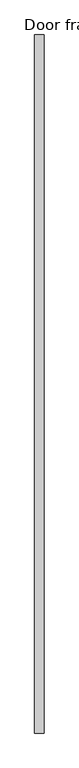
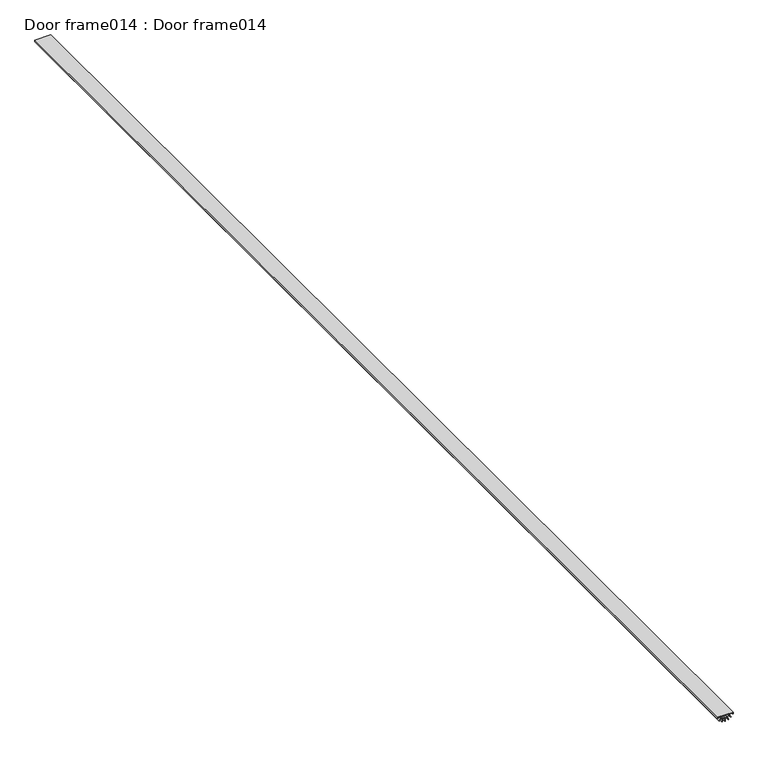
"""IFC4 building model written with IfcOpenShell, lengths in millimetres: proxy geometry, Door frame014 : Door frame014."""

import ifcopenshell
import ifcopenshell.guid

model = None  # the IFC model being written
_history = None  # IfcOwnerHistory: only IFC2X3 demands one
_inside = {}  # id of a spatial element -> (the spatial element, [elements in it])
_under = {}  # id of a project, library or spatial element -> (it, [spatial elements below it])
_declared = {}  # id of a project -> (the project, [libraries it declares])
_typed = {}  # id of a type object -> (the type object, [elements of that type])
_made_of = {}  # id of a material, layer set ... -> (it, [elements and type objects made of it])


def new_model(schema):
    """Start an empty IFC model of exactly this schema.

    Asked for "IFC4X3", IfcOpenShell would pick the latest addendum, in which some entities
    have other attributes; the version numbers below select the first issue.
    IFC2X3 requires an IfcOwnerHistory on every rooted entity: one is made here for all.
    """
    global model, _history
    if schema == "IFC4X3":
        model = ifcopenshell.file(schema_version=(4, 3, 0, 0))
    else:
        model = ifcopenshell.file(schema=schema)
    _inside.clear()
    _under.clear()
    _declared.clear()
    _typed.clear()
    _made_of.clear()
    _history = None
    if model.schema == "IFC2X3":
        org = make("IfcOrganization", Name="unknown")
        user = make(
            "IfcPersonAndOrganization",
            ThePerson=make("IfcPerson", FamilyName="unknown"),
            TheOrganization=org,
        )
        app = make(
            "IfcApplication",
            ApplicationDeveloper=org,
            Version="unknown",
            ApplicationFullName="unknown",
            ApplicationIdentifier="unknown",
        )
        _history = make(
            "IfcOwnerHistory",
            OwningUser=user,
            OwningApplication=app,
            ChangeAction="ADDED",
            CreationDate=0,
        )
    return model


def make(cls, **values):
    """One entity of the class cls with the attributes given. An attribute that is None is left unset."""
    return model.create_entity(
        cls, **{name: value for name, value in values.items() if value is not None}
    )


def rooted(cls, **values):
    """An entity with a GlobalId (a new one), such as an element, a storey or a relation."""
    return make(cls, GlobalId=ifcopenshell.guid.new(), OwnerHistory=_history, **values)


def si_unit(unit_type, name, prefix=None):
    """IfcSIUnit, for example si_unit("LENGTHUNIT", "METRE", prefix="MILLI")."""
    return make("IfcSIUnit", UnitType=unit_type, Prefix=prefix, Name=name)


def assignment(units):
    """IfcUnitAssignment: the units of a project."""
    return None if units is None else make("IfcUnitAssignment", Units=units)


def point(xyz):
    """IfcCartesianPoint."""
    return None if xyz is None else make("IfcCartesianPoint", Coordinates=xyz)


def direction(xyz):
    """IfcDirection."""
    return None if xyz is None else make("IfcDirection", DirectionRatios=xyz)


def frame(location, z_axis=None, x_axis=None):
    """IfcAxis2Placement3D, a coordinate frame: its origin and axes. An axis left out is left unset."""
    return make(
        "IfcAxis2Placement3D",
        Location=point(location),
        Axis=direction(z_axis),
        RefDirection=direction(x_axis),
    )


def origin():
    """The frame at (0, 0, 0) with its axes left unset."""
    return frame((0.0, 0.0, 0.0))


def place(relative_to, where):
    """IfcLocalPlacement: puts the frame where relative to a parent placement (None: the world)."""
    return make(
        "IfcLocalPlacement", PlacementRelTo=relative_to, RelativePlacement=where
    )


def context(
    kind, dimensions, precision=None, world=None, true_north=None, identifier=None
):
    """IfcGeometricRepresentationContext, for example the 3D "Model" context."""
    return make(
        "IfcGeometricRepresentationContext",
        ContextIdentifier=identifier,
        ContextType=kind,
        CoordinateSpaceDimension=dimensions,
        Precision=precision,
        WorldCoordinateSystem=world,
        TrueNorth=true_north,
    )


def project(units=None, contexts=None):
    """IfcProject with its units and contexts."""
    return rooted(
        "IfcProject",
        Name="project",
        RepresentationContexts=contexts,
        UnitsInContext=assignment(units),
    )


def spatial(cls, under=None, at=None, **own):
    """A site, building, storey or space (cls), placed at a placement, below another one or the project."""
    s = rooted(cls, ObjectPlacement=at, **own)
    if under is not None:
        _under.setdefault(under.id(), (under, []))[1].append(s)
    return s


def polyline(points):
    """IfcPolyline through the points."""
    return make("IfcPolyline", Points=[point(p) for p in points])


def outline(outer, holes=None, kind="AREA"):
    """IfcArbitraryClosedProfileDef: a profile drawn as a closed curve; with holes, ...WithVoids."""
    if holes is None:
        return make("IfcArbitraryClosedProfileDef", ProfileType=kind, OuterCurve=outer)
    return make(
        "IfcArbitraryProfileDefWithVoids",
        ProfileType=kind,
        OuterCurve=outer,
        InnerCurves=holes,
    )


def extrude(swept, where, along, depth):
    """IfcExtrudedAreaSolid: the profile swept, set in the frame where, extruded along a direction by depth."""
    return make(
        "IfcExtrudedAreaSolid",
        SweptArea=swept,
        Position=where,
        ExtrudedDirection=direction(along),
        Depth=depth,
    )


def shape(context_of_items, identifier, shape_type, items):
    """IfcShapeRepresentation: the items that make up one representation, for example the "Body"."""
    return make(
        "IfcShapeRepresentation",
        ContextOfItems=context_of_items,
        RepresentationIdentifier=identifier,
        RepresentationType=shape_type,
        Items=items,
    )


def source(mapping_origin, context_of_items, identifier, shape_type, items):
    """IfcRepresentationMap: a shape defined once, which mapped items show again and again."""
    return make(
        "IfcRepresentationMap",
        MappingOrigin=mapping_origin,
        MappedRepresentation=shape(context_of_items, identifier, shape_type, items),
    )


def transform(
    local_origin,
    x_axis=None,
    y_axis=None,
    z_axis=None,
    scale=None,
    scale2=None,
    scale3=None,
    uniform=True,
):
    """IfcCartesianTransformationOperator3D, or its non-uniform kind. x_axis, y_axis, z_axis: its Axis1, 2, 3."""
    if uniform:
        return make(
            "IfcCartesianTransformationOperator3D",
            Axis1=direction(x_axis),
            Axis2=direction(y_axis),
            LocalOrigin=point(local_origin),
            Scale=scale,
            Axis3=direction(z_axis),
        )
    return make(
        "IfcCartesianTransformationOperator3DnonUniform",
        Axis1=direction(x_axis),
        Axis2=direction(y_axis),
        LocalOrigin=point(local_origin),
        Scale=scale,
        Axis3=direction(z_axis),
        Scale2=scale2,
        Scale3=scale3,
    )


def mapped(mapping_source, mapping_target):
    """IfcMappedItem: shows the shape of a source again, moved by a transform."""
    return make(
        "IfcMappedItem", MappingSource=mapping_source, MappingTarget=mapping_target
    )


def made_of(thing, what):
    """Note that an element or type object is made of a material, layer set ...; save() writes the relation."""
    if what is not None:
        _made_of.setdefault(what.id(), (what, []))[1].append(thing)
    return thing


def element(
    cls,
    number,
    at=None,
    inside=None,
    cuts=None,
    type_object=None,
    material=None,
    context=None,
    identifier="Body",
    shape_type=None,
    held_by="IfcProductDefinitionShape",
    body=None,
    shapes=None,
    **own,
):
    """One element of the class cls, such as IfcWall. Its Tag is "e" and its number.

    at: its placement. inside: the storey or other place that contains it. cuts: it is an
    opening in that element (IfcRelVoidsElement). A single representation is given by context,
    identifier, shape_type and body (its items); several are given by shapes. held_by: the class
    of the entity that holds the representations. save() writes the other relations.
    """
    e = rooted(cls, Tag="e%d" % number, ObjectPlacement=at, **own)
    if body is not None:
        shapes = [shape(context, identifier, shape_type, body)]
    if shapes is not None:
        e.Representation = make(held_by, Representations=shapes)
    if inside is not None:
        _inside.setdefault(inside.id(), (inside, []))[1].append(e)
    if cuts is not None:
        rooted(
            "IfcRelVoidsElement", RelatingBuildingElement=cuts, RelatedOpeningElement=e
        )
    if type_object is not None:
        _typed.setdefault(type_object.id(), (type_object, []))[1].append(e)
    return made_of(e, material)


def aggregate(whole, parts):
    """IfcRelAggregates: a whole, such as a stair, and the parts it consists of."""
    return rooted("IfcRelAggregates", RelatingObject=whole, RelatedObjects=parts)


def save(model, path):
    """Write the relations noted so far, then the file.

    IfcRelAggregates (storeys below a building ...), IfcRelContainedInSpatialStructure (elements
    in a storey), IfcRelDefinesByType, IfcRelAssociatesMaterial and IfcRelDeclares: one each for
    every whole, place, type object, material and project.
    """
    for whole, parts in _under.values():
        aggregate(whole, parts)
    for where, things in _inside.values():
        rooted(
            "IfcRelContainedInSpatialStructure",
            RelatedElements=things,
            RelatingStructure=where,
        )
    for kind, things in _typed.values():
        rooted("IfcRelDefinesByType", RelatedObjects=things, RelatingType=kind)
    for what, things in _made_of.values():
        rooted("IfcRelAssociatesMaterial", RelatedObjects=things, RelatingMaterial=what)
    for by, libraries in _declared.values():
        rooted("IfcRelDeclares", RelatingContext=by, RelatedDefinitions=libraries)
    model.write(path)


def door_frame014_door_frame014_1e3dbea9(model_context):
    return source(origin(), model_context, "Body", "SweptSolid", [
        extrude(outline(polyline([(36578.3756733, 15524.8710245), (36578.3756733, 15525.6647745), (36583.8229098, 15525.6647745), (36584.304169, 15528.4194862), (36579.1830903, 15530.2833952), (36579.4545674, 15531.0292768), (36584.573299, 15529.166222), (36585.9800182, 15531.6205482), (36581.8052868, 15535.1235857), (36582.3155014, 15535.731632), (36586.4883159, 15532.2302029), (36588.5541303, 15533.9941318), (36588.5541303, 15536.9862907), (36587.284361, 15536.9862907), (36587.284361, 15538.6848615), (36589.8546103, 15538.6848615), (36589.8546103, 15511.5429442), (36587.284361, 15511.5429442), (36587.284361, 15513.5495083), (36588.5541303, 15513.5495083), (36588.5541303, 15516.5416672), (36586.5323252, 15518.2570371), (36582.3575787, 15514.7540195), (36581.8473669, 15515.362068), (36586.0201974, 15518.8634779), (36584.5980367, 15521.3089171), (36579.4769756, 15519.4449702), (36579.2054928, 15520.1908496), (36584.3242102, 15522.0539435), (36583.8229098, 15524.8710245), (36578.3756733, 15524.8710245)]), holes=[polyline([(36588.5541303, 15532.8858954), (36586.6136518, 15530.8738124), (36585.2069325, 15528.4194862), (36584.7256733, 15525.6647745), (36584.7256733, 15524.8710245), (36585.2269736, 15522.0539435), (36586.6491343, 15519.6085043), (36588.5541303, 15517.6499036), (36588.5541303, 15532.8858954)])]), frame((0.0, -1052.8906567, 0.0), z_axis=(0.0, 1.0, 0.0), x_axis=(0.0, 0.0, 1.0)), (0.0, 0.0, 1.0), 1999.85),
    ])


if __name__ == "__main__":
    model = new_model("IFC4")
    model_context = context("Model", 3, world=origin())
    ifc_project = project(units=[si_unit("LENGTHUNIT", "METRE", prefix="MILLI")], contexts=[model_context])
    site = spatial("IfcSite", under=ifc_project)
    building = spatial("IfcBuilding", under=site)
    placement = place(None, origin())
    door_frame014_door_frame014_shape = door_frame014_door_frame014_1e3dbea9(model_context)
    element("IfcBuildingElementProxy", 1, Name="Door frame014 : Door frame014", ObjectType="Door frame014 : Door frame014", at=placement, inside=building, context=model_context, shape_type="MappedRepresentation", body=[
        mapped(door_frame014_door_frame014_shape, transform((0.0, 0.0, 0.0), x_axis=(1.0, 0.0, 0.0), y_axis=(0.0, 1.0, 0.0), z_axis=(0.0, 0.0, 1.0))),
    ])
    save(model, "model.ifc")

# Revit data of these elements
# Type "Door frame014 : Door frame014"
#   NameOverride = "Door frame014"
# Element 1 (IfcBuildingElementProxy, "Door frame014 : Door frame014")
#   Materials on its faces: "WEATHERSTRIPPING SWEEP"
# Materials
#   "WEATHERSTRIPPING SWEEP": class "Wood", colour RGB 212 179 113, transparency 0, Description = "Plywood, sheathing grade", Cost = 0
